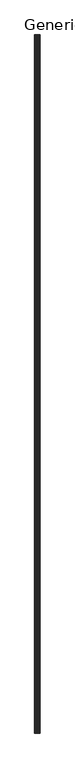
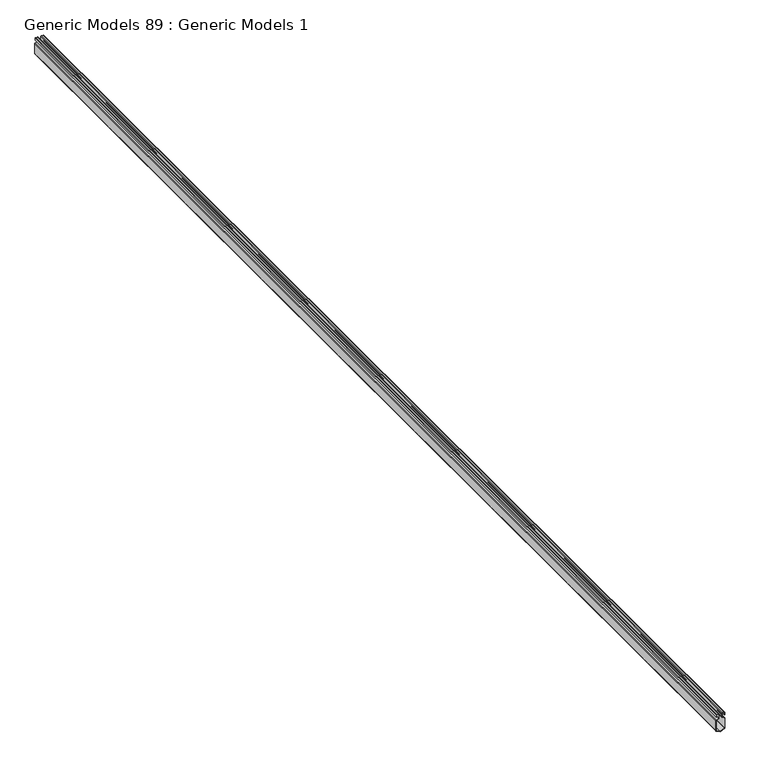
"""IFC4 building model written with IfcOpenShell, lengths in millimetres: proxy geometry, Generic Models 89 : Generic Models 1."""

from ifc_helpers import new_model, si_unit, point, frame, frame_2d, origin, place, context, project, spatial, polyline, circle_curve, trimmed, segment, composite_curve, outline, extrude, source, transform, mapped, element, save


def generic_models_89_generic_models_1_039e3ccd(model_context):
    return source(origin(), model_context, "Body", "SweptSolid", [
        extrude(outline(composite_curve([segment(trimmed(circle_curve(frame_2d((123087.1594358, -10108.6422218)), 1.5875), [point((123088.7469358, -10108.6422218))], [point((123087.1594358, -10107.0547218))], True, "CARTESIAN"), True, "CONTINUOUS"), segment(polyline([(123087.1594358, -10107.0547218), (123071.5943158, -10107.0547218), (123071.5943158, -10105.1573418), (123087.4693158, -10105.1573418)]), True, "CONTINUOUS"), segment(trimmed(circle_curve(frame_2d((123087.4693158, -10108.3323418)), 3.175), [point((123087.4693158, -10105.1573418))], [point((123090.6443158, -10108.3323418))], False, "CARTESIAN"), True, "CONTINUOUS"), segment(polyline([(123090.6443158, -10108.3323418), (123090.6443158, -10121.0323418)]), True, "CONTINUOUS"), segment(trimmed(circle_curve(frame_2d((123087.4693158, -10121.0323418)), 3.175), [point((123090.6443158, -10121.0323418))], [point((123087.4693158, -10124.2073418))], False, "CARTESIAN"), True, "CONTINUOUS"), segment(polyline([(123087.4693158, -10124.2073418), (123060.7981683, -10124.2073418)]), True, "CONTINUOUS"), segment(trimmed(circle_curve(frame_2d((123060.7981683, -10121.0323418)), 3.175), [point((123060.7981683, -10124.2073418))], [point((123057.9974924, -10122.5279484))], False, "CARTESIAN"), True, "CONTINUOUS"), segment(polyline([(123057.9974924, -10122.5279484), (123049.5311385, -10106.6738377)]), True, "CONTINUOUS"), segment(trimmed(circle_curve(frame_2d((123048.1308005, -10107.421641)), 1.5875), [point((123049.5311385, -10106.6738377))], [point((123048.1308005, -10105.834141))], True, "CARTESIAN"), True, "CONTINUOUS"), segment(polyline([(123048.1308005, -10105.834141), (122977.2538938, -10105.834141)]), True, "CONTINUOUS"), segment(trimmed(circle_curve(frame_2d((122977.2538938, -10107.421641)), 1.5875), [point((122977.2538938, -10105.834141))], [point((122975.7976254, -10106.7896295))], True, "CARTESIAN"), True, "CONTINUOUS"), segment(polyline([(122975.7976254, -10106.7896295), (122963.791686, -10134.4534806), (122977.2929532, -10161.4861982)]), True, "CONTINUOUS"), segment(trimmed(circle_curve(frame_2d((122978.7131733, -10160.776881)), 1.5875), [point((122977.2929532, -10161.4861982))], [point((122978.7131733, -10162.364381))], True, "CARTESIAN"), True, "CONTINUOUS"), segment(polyline([(122978.7131733, -10162.364381), (123049.5603872, -10162.364381)]), True, "CONTINUOUS"), segment(trimmed(circle_curve(frame_2d((123049.5603872, -10160.776881)), 1.5875), [point((123049.5603872, -10162.364381))], [point((123051.0166557, -10161.4088924))], True, "CARTESIAN"), True, "CONTINUOUS"), segment(polyline([(123051.0166557, -10161.4088924), (123058.0649636, -10145.1683189)]), True, "CONTINUOUS"), segment(trimmed(circle_curve(frame_2d((123060.9775005, -10146.4323418)), 3.175), [point((123058.0649636, -10145.1683189))], [point((123060.9775005, -10143.2573418))], False, "CARTESIAN"), True, "CONTINUOUS"), segment(polyline([(123060.9775005, -10143.2573418), (123087.4693158, -10143.2573418)]), True, "CONTINUOUS"), segment(trimmed(circle_curve(frame_2d((123087.4693158, -10146.4323418)), 3.175), [point((123087.4693158, -10143.2573418))], [point((123090.6443158, -10146.4323418))], False, "CARTESIAN"), True, "CONTINUOUS"), segment(polyline([(123090.6443158, -10146.4323418), (123090.6443158, -10159.1323418)]), True, "CONTINUOUS"), segment(trimmed(circle_curve(frame_2d((123087.4693158, -10159.1323418)), 3.175), [point((123090.6443158, -10159.1323418))], [point((123087.4693158, -10162.3073418))], False, "CARTESIAN"), True, "CONTINUOUS"), segment(polyline([(123087.4693158, -10162.3073418), (123071.5943158, -10162.3073418), (123071.5943158, -10160.4099618), (123087.1594358, -10160.4099618)]), True, "CONTINUOUS"), segment(trimmed(circle_curve(frame_2d((123087.1594358, -10158.8224618)), 1.5875), [point((123087.1594358, -10160.4099618))], [point((123088.7469358, -10158.8224618))], True, "CARTESIAN"), True, "CONTINUOUS"), segment(polyline([(123088.7469358, -10158.8224618), (123088.7469358, -10146.7422218)]), True, "CONTINUOUS"), segment(trimmed(circle_curve(frame_2d((123087.1594358, -10146.7422218)), 1.5875), [point((123088.7469358, -10146.7422218))], [point((123087.1594358, -10145.1547218))], True, "CARTESIAN"), True, "CONTINUOUS"), segment(polyline([(123087.1594358, -10145.1547218), (123061.1808193, -10145.1547218)]), True, "CONTINUOUS"), segment(trimmed(circle_curve(frame_2d((123061.1808193, -10146.7422218)), 1.5875), [point((123061.1808193, -10145.1547218))], [point((123059.7245509, -10146.1102103))], True, "CARTESIAN"), True, "CONTINUOUS"), segment(polyline([(123059.7245509, -10146.1102103), (123052.6762429, -10162.3507839)]), True, "CONTINUOUS"), segment(trimmed(circle_curve(frame_2d((123049.763706, -10161.086761)), 3.175), [point((123052.6762429, -10162.3507839))], [point((123049.763706, -10164.261761))], False, "CARTESIAN"), True, "CONTINUOUS"), segment(polyline([(123049.763706, -10164.261761), (122978.5215613, -10164.261761)]), True, "CONTINUOUS"), segment(trimmed(circle_curve(frame_2d((122978.5215613, -10161.086761)), 3.175), [point((122978.5215613, -10164.261761))], [point((122975.6811209, -10162.5053954))], False, "CARTESIAN"), True, "CONTINUOUS"), segment(polyline([(122975.6811209, -10162.5053954), (122961.6989144, -10134.5097239), (122974.1380381, -10105.8477381)]), True, "CONTINUOUS"), segment(trimmed(circle_curve(frame_2d((122977.050575, -10107.111761)), 3.175), [point((122974.1380381, -10105.8477381))], [point((122977.050575, -10103.936761))], False, "CARTESIAN"), True, "CONTINUOUS"), segment(polyline([(122977.050575, -10103.936761), (123048.3166165, -10103.936761)]), True, "CONTINUOUS"), segment(trimmed(circle_curve(frame_2d((123048.3166165, -10107.111761)), 3.175), [point((123048.3166165, -10103.936761))], [point((123051.1172924, -10105.6161543))], False, "CARTESIAN"), True, "CONTINUOUS"), segment(polyline([(123051.1172924, -10105.6161543), (123059.5836463, -10121.4702651)]), True, "CONTINUOUS"), segment(trimmed(circle_curve(frame_2d((123060.9839843, -10120.7224618)), 1.5875), [point((123059.5836463, -10121.4702651))], [point((123060.9839843, -10122.3099618))], True, "CARTESIAN"), True, "CONTINUOUS"), segment(polyline([(123060.9839843, -10122.3099618), (123087.1594358, -10122.3099618)]), True, "CONTINUOUS"), segment(trimmed(circle_curve(frame_2d((123087.1594358, -10120.7224618)), 1.5875), [point((123087.1594358, -10122.3099618))], [point((123088.7469358, -10120.7224618))], True, "CARTESIAN"), True, "CONTINUOUS"), segment(polyline([(123088.7469358, -10120.7224618), (123088.7469358, -10108.6422218)]), True, "CONTINUOUS")], self_intersect=False)), frame((0.0, -5493.3230338, 0.0), z_axis=(0.0, 1.0, 0.0), x_axis=(0.0, 0.0, 1.0)), (0.0, 0.0, 1.0), 7886.7),
    ])


if __name__ == "__main__":
    model = new_model("IFC4")
    model_context = context("Model", 3, world=origin())
    ifc_project = project(units=[si_unit("LENGTHUNIT", "METRE", prefix="MILLI")], contexts=[model_context])
    site = spatial("IfcSite", under=ifc_project)
    building = spatial("IfcBuilding", under=site)
    placement = place(None, origin())
    generic_models_89_generic_models_1_shape = generic_models_89_generic_models_1_039e3ccd(model_context)
    element("IfcBuildingElementProxy", 1, Name="Generic Models 89 : Generic Models 1", ObjectType="Generic Models 89 : Generic Models 1", at=placement, inside=building, context=model_context, shape_type="MappedRepresentation", body=[
        mapped(generic_models_89_generic_models_1_shape, transform((0.0, 0.0, 0.0), x_axis=(1.0, 0.0, 0.0), y_axis=(0.0, 1.0, 0.0), z_axis=(0.0, 0.0, 1.0))),
    ])
    save(model, "model.ifc")

# Revit data of these elements
# Element 1 (IfcBuildingElementProxy, "Generic Models 89 : Generic Models 1")
#   Materials on its faces: "_SS SLOT DRAIN -  Z891 SANI-FLO"
# Materials
#   "_SS SLOT DRAIN -  Z891 SANI-FLO": class "Generic", colour RGB 253 192 103, transparency 0, Cost = 0
